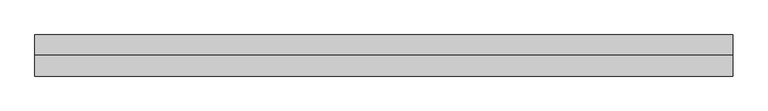
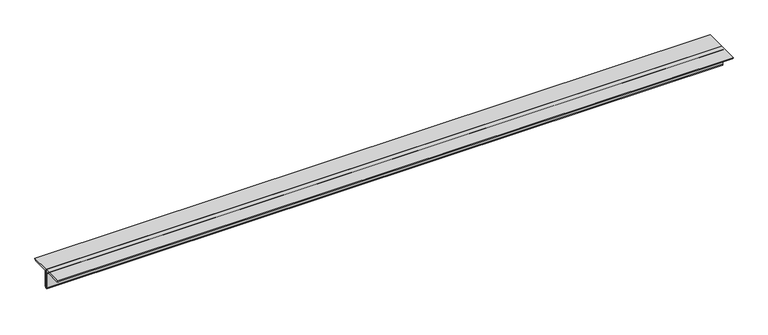
"""IFC4 building model written with IfcOpenShell, lengths in millimetres: member geometry, 0123_Steel Framing_2Ls-KSD3502 : H_SB_AR_S03_2Ls-130x130x12_HBR1."""

import ifcopenshell
import ifcopenshell.guid

model = None  # the IFC model being written
_history = None  # IfcOwnerHistory: only IFC2X3 demands one
_inside = {}  # id of a spatial element -> (the spatial element, [elements in it])
_under = {}  # id of a project, library or spatial element -> (it, [spatial elements below it])
_declared = {}  # id of a project -> (the project, [libraries it declares])
_typed = {}  # id of a type object -> (the type object, [elements of that type])
_made_of = {}  # id of a material, layer set ... -> (it, [elements and type objects made of it])


def new_model(schema):
    """Start an empty IFC model of exactly this schema.

    Asked for "IFC4X3", IfcOpenShell would pick the latest addendum, in which some entities
    have other attributes; the version numbers below select the first issue.
    IFC2X3 requires an IfcOwnerHistory on every rooted entity: one is made here for all.
    """
    global model, _history
    if schema == "IFC4X3":
        model = ifcopenshell.file(schema_version=(4, 3, 0, 0))
    else:
        model = ifcopenshell.file(schema=schema)
    _inside.clear()
    _under.clear()
    _declared.clear()
    _typed.clear()
    _made_of.clear()
    _history = None
    if model.schema == "IFC2X3":
        org = make("IfcOrganization", Name="unknown")
        user = make(
            "IfcPersonAndOrganization",
            ThePerson=make("IfcPerson", FamilyName="unknown"),
            TheOrganization=org,
        )
        app = make(
            "IfcApplication",
            ApplicationDeveloper=org,
            Version="unknown",
            ApplicationFullName="unknown",
            ApplicationIdentifier="unknown",
        )
        _history = make(
            "IfcOwnerHistory",
            OwningUser=user,
            OwningApplication=app,
            ChangeAction="ADDED",
            CreationDate=0,
        )
    return model


def make(cls, **values):
    """One entity of the class cls with the attributes given. An attribute that is None is left unset."""
    return model.create_entity(
        cls, **{name: value for name, value in values.items() if value is not None}
    )


def rooted(cls, **values):
    """An entity with a GlobalId (a new one), such as an element, a storey or a relation."""
    return make(cls, GlobalId=ifcopenshell.guid.new(), OwnerHistory=_history, **values)


def si_unit(unit_type, name, prefix=None):
    """IfcSIUnit, for example si_unit("LENGTHUNIT", "METRE", prefix="MILLI")."""
    return make("IfcSIUnit", UnitType=unit_type, Prefix=prefix, Name=name)


def assignment(units):
    """IfcUnitAssignment: the units of a project."""
    return None if units is None else make("IfcUnitAssignment", Units=units)


def point(xyz):
    """IfcCartesianPoint."""
    return None if xyz is None else make("IfcCartesianPoint", Coordinates=xyz)


def direction(xyz):
    """IfcDirection."""
    return None if xyz is None else make("IfcDirection", DirectionRatios=xyz)


def frame(location, z_axis=None, x_axis=None):
    """IfcAxis2Placement3D, a coordinate frame: its origin and axes. An axis left out is left unset."""
    return make(
        "IfcAxis2Placement3D",
        Location=point(location),
        Axis=direction(z_axis),
        RefDirection=direction(x_axis),
    )


def frame_2d(location, x_axis=None):
    """IfcAxis2Placement2D, a coordinate frame in the plane: its origin and x axis."""
    return make(
        "IfcAxis2Placement2D", Location=point(location), RefDirection=direction(x_axis)
    )


def origin():
    """The frame at (0, 0, 0) with its axes left unset."""
    return frame((0.0, 0.0, 0.0))


def place(relative_to, where):
    """IfcLocalPlacement: puts the frame where relative to a parent placement (None: the world)."""
    return make(
        "IfcLocalPlacement", PlacementRelTo=relative_to, RelativePlacement=where
    )


def context(
    kind, dimensions, precision=None, world=None, true_north=None, identifier=None
):
    """IfcGeometricRepresentationContext, for example the 3D "Model" context."""
    return make(
        "IfcGeometricRepresentationContext",
        ContextIdentifier=identifier,
        ContextType=kind,
        CoordinateSpaceDimension=dimensions,
        Precision=precision,
        WorldCoordinateSystem=world,
        TrueNorth=true_north,
    )


def project(units=None, contexts=None):
    """IfcProject with its units and contexts."""
    return rooted(
        "IfcProject",
        Name="project",
        RepresentationContexts=contexts,
        UnitsInContext=assignment(units),
    )


def spatial(cls, under=None, at=None, **own):
    """A site, building, storey or space (cls), placed at a placement, below another one or the project."""
    s = rooted(cls, ObjectPlacement=at, **own)
    if under is not None:
        _under.setdefault(under.id(), (under, []))[1].append(s)
    return s


def polyline(points):
    """IfcPolyline through the points."""
    return make("IfcPolyline", Points=[point(p) for p in points])


def circle_curve(where, radius):
    """IfcCircle in the frame where."""
    return make("IfcCircle", Position=where, Radius=radius)


def trimmed(basis, trim1, trim2, sense, master):
    """IfcTrimmedCurve: the piece of a basis curve between two trims."""
    return make(
        "IfcTrimmedCurve",
        BasisCurve=basis,
        Trim1=trim1,
        Trim2=trim2,
        SenseAgreement=sense,
        MasterRepresentation=master,
    )


def segment(curve, same_sense, transition):
    """IfcCompositeCurveSegment."""
    return make(
        "IfcCompositeCurveSegment",
        Transition=transition,
        SameSense=same_sense,
        ParentCurve=curve,
    )


def composite_curve(segments, self_intersect=None):
    """IfcCompositeCurve: segments joined end to end."""
    return make("IfcCompositeCurve", Segments=segments, SelfIntersect=self_intersect)


def outline(outer, holes=None, kind="AREA"):
    """IfcArbitraryClosedProfileDef: a profile drawn as a closed curve; with holes, ...WithVoids."""
    if holes is None:
        return make("IfcArbitraryClosedProfileDef", ProfileType=kind, OuterCurve=outer)
    return make(
        "IfcArbitraryProfileDefWithVoids",
        ProfileType=kind,
        OuterCurve=outer,
        InnerCurves=holes,
    )


def extrude(swept, where, along, depth):
    """IfcExtrudedAreaSolid: the profile swept, set in the frame where, extruded along a direction by depth."""
    return make(
        "IfcExtrudedAreaSolid",
        SweptArea=swept,
        Position=where,
        ExtrudedDirection=direction(along),
        Depth=depth,
    )


def shape(context_of_items, identifier, shape_type, items):
    """IfcShapeRepresentation: the items that make up one representation, for example the "Body"."""
    return make(
        "IfcShapeRepresentation",
        ContextOfItems=context_of_items,
        RepresentationIdentifier=identifier,
        RepresentationType=shape_type,
        Items=items,
    )


def source(mapping_origin, context_of_items, identifier, shape_type, items):
    """IfcRepresentationMap: a shape defined once, which mapped items show again and again."""
    return make(
        "IfcRepresentationMap",
        MappingOrigin=mapping_origin,
        MappedRepresentation=shape(context_of_items, identifier, shape_type, items),
    )


def transform(
    local_origin,
    x_axis=None,
    y_axis=None,
    z_axis=None,
    scale=None,
    scale2=None,
    scale3=None,
    uniform=True,
):
    """IfcCartesianTransformationOperator3D, or its non-uniform kind. x_axis, y_axis, z_axis: its Axis1, 2, 3."""
    if uniform:
        return make(
            "IfcCartesianTransformationOperator3D",
            Axis1=direction(x_axis),
            Axis2=direction(y_axis),
            LocalOrigin=point(local_origin),
            Scale=scale,
            Axis3=direction(z_axis),
        )
    return make(
        "IfcCartesianTransformationOperator3DnonUniform",
        Axis1=direction(x_axis),
        Axis2=direction(y_axis),
        LocalOrigin=point(local_origin),
        Scale=scale,
        Axis3=direction(z_axis),
        Scale2=scale2,
        Scale3=scale3,
    )


def mapped(mapping_source, mapping_target):
    """IfcMappedItem: shows the shape of a source again, moved by a transform."""
    return make(
        "IfcMappedItem", MappingSource=mapping_source, MappingTarget=mapping_target
    )


def made_of(thing, what):
    """Note that an element or type object is made of a material, layer set ...; save() writes the relation."""
    if what is not None:
        _made_of.setdefault(what.id(), (what, []))[1].append(thing)
    return thing


def element(
    cls,
    number,
    at=None,
    inside=None,
    cuts=None,
    type_object=None,
    material=None,
    context=None,
    identifier="Body",
    shape_type=None,
    held_by="IfcProductDefinitionShape",
    body=None,
    shapes=None,
    **own,
):
    """One element of the class cls, such as IfcWall. Its Tag is "e" and its number.

    at: its placement. inside: the storey or other place that contains it. cuts: it is an
    opening in that element (IfcRelVoidsElement). A single representation is given by context,
    identifier, shape_type and body (its items); several are given by shapes. held_by: the class
    of the entity that holds the representations. save() writes the other relations.
    """
    e = rooted(cls, Tag="e%d" % number, ObjectPlacement=at, **own)
    if body is not None:
        shapes = [shape(context, identifier, shape_type, body)]
    if shapes is not None:
        e.Representation = make(held_by, Representations=shapes)
    if inside is not None:
        _inside.setdefault(inside.id(), (inside, []))[1].append(e)
    if cuts is not None:
        rooted(
            "IfcRelVoidsElement", RelatingBuildingElement=cuts, RelatedOpeningElement=e
        )
    if type_object is not None:
        _typed.setdefault(type_object.id(), (type_object, []))[1].append(e)
    return made_of(e, material)


def aggregate(whole, parts):
    """IfcRelAggregates: a whole, such as a stair, and the parts it consists of."""
    return rooted("IfcRelAggregates", RelatingObject=whole, RelatedObjects=parts)


def save(model, path):
    """Write the relations noted so far, then the file.

    IfcRelAggregates (storeys below a building ...), IfcRelContainedInSpatialStructure (elements
    in a storey), IfcRelDefinesByType, IfcRelAssociatesMaterial and IfcRelDeclares: one each for
    every whole, place, type object, material and project.
    """
    for whole, parts in _under.values():
        aggregate(whole, parts)
    for where, things in _inside.values():
        rooted(
            "IfcRelContainedInSpatialStructure",
            RelatedElements=things,
            RelatingStructure=where,
        )
    for kind, things in _typed.values():
        rooted("IfcRelDefinesByType", RelatedObjects=things, RelatingType=kind)
    for what, things in _made_of.values():
        rooted("IfcRelAssociatesMaterial", RelatedObjects=things, RelatingMaterial=what)
    for by, libraries in _declared.values():
        rooted("IfcRelDeclares", RelatingContext=by, RelatedDefinitions=libraries)
    model.write(path)


def member_bcbd117d(model_context):
    return source(origin(), model_context, "Body", "SweptSolid", [
        extrude(outline(composite_curve([segment(polyline([(0.0, 36.4), (0.0, -93.6)]), True, "CONTINUOUS"), segment(trimmed(circle_curve(frame_2d((0.0, -81.6)), 12.0), [point((0.0, -93.6))], [point((-12.0, -81.6))], False, "CARTESIAN"), True, "CONTINUOUS"), segment(polyline([(-12.0, -81.6), (-12.0, 12.4)]), True, "CONTINUOUS"), segment(trimmed(circle_curve(frame_2d((-24.0, 12.4)), 12.0), [point((-12.0, 12.4))], [point((-24.0, 24.4))], True, "CARTESIAN"), True, "CONTINUOUS"), segment(polyline([(-24.0, 24.4), (-118.0, 24.4)]), True, "CONTINUOUS"), segment(trimmed(circle_curve(frame_2d((-118.0, 36.4)), 12.0), [point((-118.0, 24.4))], [point((-130.0, 36.4))], False, "CARTESIAN"), True, "CONTINUOUS"), segment(polyline([(-130.0, 36.4), (0.0, 36.4)]), True, "CONTINUOUS")], self_intersect=False)), frame((-2209.5676318, 0.0, 0.0), z_axis=(1.0, 0.0, 0.0), x_axis=(0.0, 1.0, 0.0)), (0.0, 0.0, 1.0), 4412.2019305),
        extrude(outline(composite_curve([segment(polyline([(0.0, 36.4), (130.0, 36.4)]), True, "CONTINUOUS"), segment(trimmed(circle_curve(frame_2d((118.0, 36.4)), 12.0), [point((130.0, 36.4))], [point((118.0, 24.4))], False, "CARTESIAN"), True, "CONTINUOUS"), segment(polyline([(118.0, 24.4), (24.0, 24.4)]), True, "CONTINUOUS"), segment(trimmed(circle_curve(frame_2d((24.0, 12.4)), 12.0), [point((24.0, 24.4))], [point((12.0, 12.4))], True, "CARTESIAN"), True, "CONTINUOUS"), segment(polyline([(12.0, 12.4), (12.0, -81.6)]), True, "CONTINUOUS"), segment(trimmed(circle_curve(frame_2d((0.0, -81.6)), 12.0), [point((12.0, -81.6))], [point((0.0, -93.6))], False, "CARTESIAN"), True, "CONTINUOUS"), segment(polyline([(0.0, -93.6), (0.0, 36.4)]), True, "CONTINUOUS")], self_intersect=False)), frame((-2209.5676318, 0.0, 0.0), z_axis=(1.0, 0.0, 0.0), x_axis=(0.0, 1.0, 0.0)), (0.0, 0.0, 1.0), 4412.2019305),
    ])


if __name__ == "__main__":
    model = new_model("IFC4")
    model_context = context("Model", 3, world=origin())
    ifc_project = project(units=[si_unit("LENGTHUNIT", "METRE", prefix="MILLI")], contexts=[model_context])
    site = spatial("IfcSite", under=ifc_project)
    building = spatial("IfcBuilding", under=site)
    placement = place(None, origin())
    member_shape = member_bcbd117d(model_context)
    element("IfcMember", 1, ObjectType="0123_Steel Framing_2Ls-KSD3502 : H_SB_AR_S03_2Ls-130x130x12_HBR1", at=placement, inside=building, context=model_context, shape_type="MappedRepresentation", body=[
        mapped(member_shape, transform((0.0, 0.0, 0.0), x_axis=(1.0, 0.0, 0.0), y_axis=(0.0, 1.0, 0.0), z_axis=(0.0, 0.0, 1.0))),
    ])
    save(model, "model.ifc")

# Revit data of these elements
# Type "0123_Steel Framing_2Ls-KSD3502 : H_SB_AR_S03_2Ls-130x130x12_HBR1"
#   Type Mark = "HBR1"
#   Assembly Code = "B10"
#   Legs = "SLBB"
#   W = 8.97
#   Perimeter = 1.04 m²/m
#   Nominal Weight = 46.80 kgf/m
#   Length [instance default] = 1000 mm
#   Space = 0 mm
#   b = 130 mm
#   d = 130 mm
#   t = 12 mm
#   y = 36.4 mm
#   A = 0.005952 m²
#   Structural Material [instance default] = Steel ASTM A36
# Element 1 (IfcMember, "0123_Steel Framing_2Ls-KSD3502 : H_SB_AR_S03_2Ls-130x130x12_HBR1")
#   Materials on its faces: "Steel ASTM A36"
# Materials
#   "Steel ASTM A36": class "Metal", colour RGB 199 199 199, transparency 0, Description = "Structural steel, ASTM A36 Grade B, mill finish", Cost = 0
